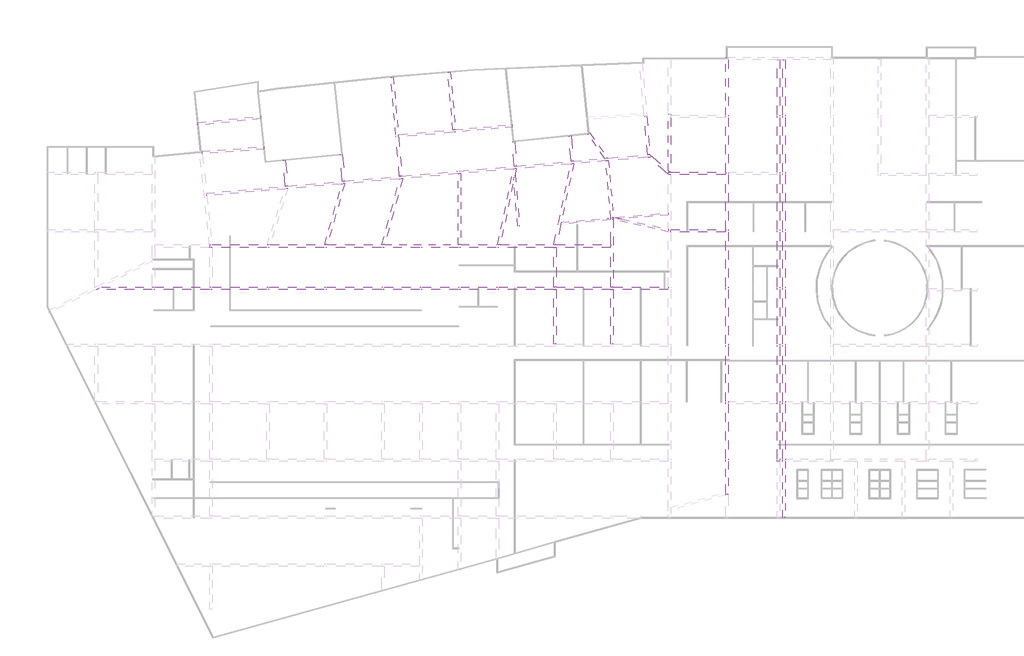
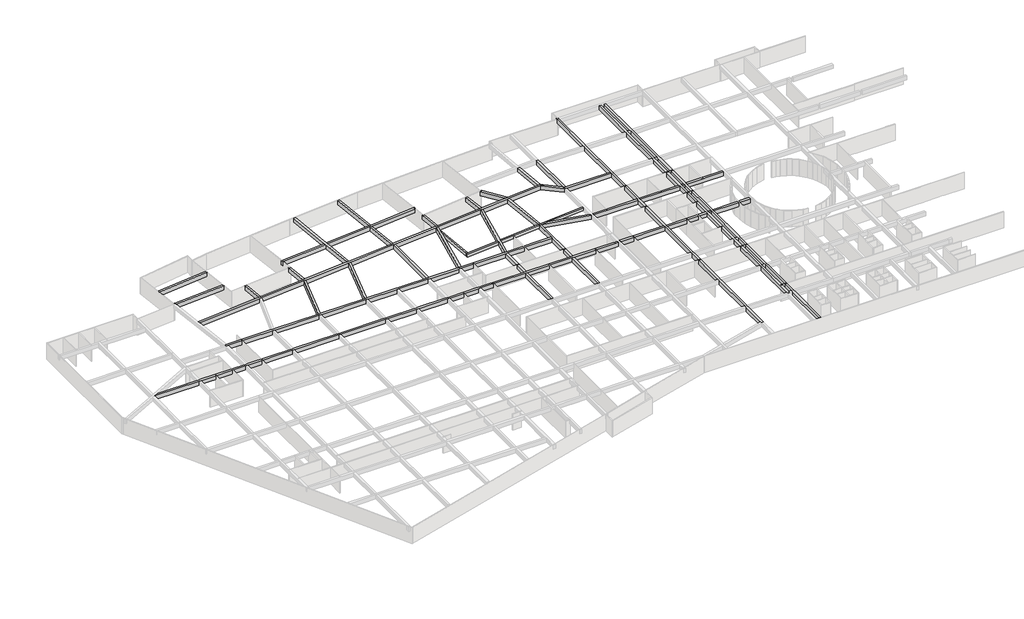
# One storey, part 7 of 8: 34 beams.
"""IFC4 building model written with IfcOpenShell, lengths in millimetres."""

import ifcopenshell
import ifcopenshell.guid

model = None  # the IFC model being written
_history = None  # IfcOwnerHistory: only IFC2X3 demands one
_inside = {}  # id of a spatial element -> (the spatial element, [elements in it])
_under = {}  # id of a project, library or spatial element -> (it, [spatial elements below it])
_declared = {}  # id of a project -> (the project, [libraries it declares])
_typed = {}  # id of a type object -> (the type object, [elements of that type])
_made_of = {}  # id of a material, layer set ... -> (it, [elements and type objects made of it])


def new_model(schema):
    """Start an empty IFC model of exactly this schema.

    Asked for "IFC4X3", IfcOpenShell would pick the latest addendum, in which some entities
    have other attributes; the version numbers below select the first issue.
    IFC2X3 requires an IfcOwnerHistory on every rooted entity: one is made here for all.
    """
    global model, _history
    if schema == "IFC4X3":
        model = ifcopenshell.file(schema_version=(4, 3, 0, 0))
    else:
        model = ifcopenshell.file(schema=schema)
    _inside.clear()
    _under.clear()
    _declared.clear()
    _typed.clear()
    _made_of.clear()
    _history = None
    if model.schema == "IFC2X3":
        org = make("IfcOrganization", Name="unknown")
        user = make(
            "IfcPersonAndOrganization",
            ThePerson=make("IfcPerson", FamilyName="unknown"),
            TheOrganization=org,
        )
        app = make(
            "IfcApplication",
            ApplicationDeveloper=org,
            Version="unknown",
            ApplicationFullName="unknown",
            ApplicationIdentifier="unknown",
        )
        _history = make(
            "IfcOwnerHistory",
            OwningUser=user,
            OwningApplication=app,
            ChangeAction="ADDED",
            CreationDate=0,
        )
    return model


def make(cls, **values):
    """One entity of the class cls with the attributes given. An attribute that is None is left unset."""
    return model.create_entity(
        cls, **{name: value for name, value in values.items() if value is not None}
    )


def rooted(cls, **values):
    """An entity with a GlobalId (a new one), such as an element, a storey or a relation."""
    return make(cls, GlobalId=ifcopenshell.guid.new(), OwnerHistory=_history, **values)


def si_unit(unit_type, name, prefix=None):
    """IfcSIUnit, for example si_unit("LENGTHUNIT", "METRE", prefix="MILLI")."""
    return make("IfcSIUnit", UnitType=unit_type, Prefix=prefix, Name=name)


def assignment(units):
    """IfcUnitAssignment: the units of a project."""
    return None if units is None else make("IfcUnitAssignment", Units=units)


def point(xyz):
    """IfcCartesianPoint."""
    return None if xyz is None else make("IfcCartesianPoint", Coordinates=xyz)


def direction(xyz):
    """IfcDirection."""
    return None if xyz is None else make("IfcDirection", DirectionRatios=xyz)


def frame(location, z_axis=None, x_axis=None):
    """IfcAxis2Placement3D, a coordinate frame: its origin and axes. An axis left out is left unset."""
    return make(
        "IfcAxis2Placement3D",
        Location=point(location),
        Axis=direction(z_axis),
        RefDirection=direction(x_axis),
    )


def origin():
    """The frame at (0, 0, 0) with its axes left unset."""
    return frame((0.0, 0.0, 0.0))


def place(relative_to, where):
    """IfcLocalPlacement: puts the frame where relative to a parent placement (None: the world)."""
    return make(
        "IfcLocalPlacement", PlacementRelTo=relative_to, RelativePlacement=where
    )


def context(
    kind, dimensions, precision=None, world=None, true_north=None, identifier=None
):
    """IfcGeometricRepresentationContext, for example the 3D "Model" context."""
    return make(
        "IfcGeometricRepresentationContext",
        ContextIdentifier=identifier,
        ContextType=kind,
        CoordinateSpaceDimension=dimensions,
        Precision=precision,
        WorldCoordinateSystem=world,
        TrueNorth=true_north,
    )


def project(units=None, contexts=None):
    """IfcProject with its units and contexts."""
    return rooted(
        "IfcProject",
        Name="project",
        RepresentationContexts=contexts,
        UnitsInContext=assignment(units),
    )


def spatial(cls, under=None, at=None, **own):
    """A site, building, storey or space (cls), placed at a placement, below another one or the project."""
    s = rooted(cls, ObjectPlacement=at, **own)
    if under is not None:
        _under.setdefault(under.id(), (under, []))[1].append(s)
    return s


def polyline(points):
    """IfcPolyline through the points."""
    return make("IfcPolyline", Points=[point(p) for p in points])


def outline(outer, holes=None, kind="AREA"):
    """IfcArbitraryClosedProfileDef: a profile drawn as a closed curve; with holes, ...WithVoids."""
    if holes is None:
        return make("IfcArbitraryClosedProfileDef", ProfileType=kind, OuterCurve=outer)
    return make(
        "IfcArbitraryProfileDefWithVoids",
        ProfileType=kind,
        OuterCurve=outer,
        InnerCurves=holes,
    )


def extrude(swept, where, along, depth):
    """IfcExtrudedAreaSolid: the profile swept, set in the frame where, extruded along a direction by depth."""
    return make(
        "IfcExtrudedAreaSolid",
        SweptArea=swept,
        Position=where,
        ExtrudedDirection=direction(along),
        Depth=depth,
    )


def faces_of(points, faces, orient=None, outer=None):
    """IfcFace entities. A face is a list of loops; a loop is a list of indices into points, from 0.

    orient and outer hold one flag for each loop. By default every Orientation is true, the
    first loop of a face is its IfcFaceOuterBound and the others are IfcFaceBound.
    """
    made = []
    for i, loops in enumerate(faces):
        bounds = []
        for j, loop in enumerate(loops):
            is_outer = j == 0 if outer is None else outer[i][j]
            bounds.append(
                make(
                    "IfcFaceOuterBound" if is_outer else "IfcFaceBound",
                    Bound=make("IfcPolyLoop", Polygon=[points[k] for k in loop]),
                    Orientation=True if orient is None else orient[i][j],
                )
            )
        made.append(make("IfcFace", Bounds=bounds))
    return made


def faceted_brep(points, faces, orient=None, outer=None, voids=None):
    """IfcFacetedBrep: a solid bounded by flat faces; with voids (closed shells), ...WithVoids."""
    shared = [point(p) for p in points]
    hull = make("IfcClosedShell", CfsFaces=faces_of(shared, faces, orient, outer))
    if voids is None:
        return make("IfcFacetedBrep", Outer=hull)
    return make(
        "IfcFacetedBrepWithVoids",
        Outer=hull,
        Voids=[
            make(cls, CfsFaces=faces_of(shared, fs, o, b)) for cls, fs, o, b in voids
        ],
    )


def shape(context_of_items, identifier, shape_type, items):
    """IfcShapeRepresentation: the items that make up one representation, for example the "Body"."""
    return make(
        "IfcShapeRepresentation",
        ContextOfItems=context_of_items,
        RepresentationIdentifier=identifier,
        RepresentationType=shape_type,
        Items=items,
    )


def source(mapping_origin, context_of_items, identifier, shape_type, items):
    """IfcRepresentationMap: a shape defined once, which mapped items show again and again."""
    return make(
        "IfcRepresentationMap",
        MappingOrigin=mapping_origin,
        MappedRepresentation=shape(context_of_items, identifier, shape_type, items),
    )


def transform(
    local_origin,
    x_axis=None,
    y_axis=None,
    z_axis=None,
    scale=None,
    scale2=None,
    scale3=None,
    uniform=True,
):
    """IfcCartesianTransformationOperator3D, or its non-uniform kind. x_axis, y_axis, z_axis: its Axis1, 2, 3."""
    if uniform:
        return make(
            "IfcCartesianTransformationOperator3D",
            Axis1=direction(x_axis),
            Axis2=direction(y_axis),
            LocalOrigin=point(local_origin),
            Scale=scale,
            Axis3=direction(z_axis),
        )
    return make(
        "IfcCartesianTransformationOperator3DnonUniform",
        Axis1=direction(x_axis),
        Axis2=direction(y_axis),
        LocalOrigin=point(local_origin),
        Scale=scale,
        Axis3=direction(z_axis),
        Scale2=scale2,
        Scale3=scale3,
    )


def mapped(mapping_source, mapping_target):
    """IfcMappedItem: shows the shape of a source again, moved by a transform."""
    return make(
        "IfcMappedItem", MappingSource=mapping_source, MappingTarget=mapping_target
    )


def made_of(thing, what):
    """Note that an element or type object is made of a material, layer set ...; save() writes the relation."""
    if what is not None:
        _made_of.setdefault(what.id(), (what, []))[1].append(thing)
    return thing


def element(
    cls,
    number,
    at=None,
    inside=None,
    cuts=None,
    type_object=None,
    material=None,
    context=None,
    identifier="Body",
    shape_type=None,
    held_by="IfcProductDefinitionShape",
    body=None,
    shapes=None,
    **own,
):
    """One element of the class cls, such as IfcWall. Its Tag is "e" and its number.

    at: its placement. inside: the storey or other place that contains it. cuts: it is an
    opening in that element (IfcRelVoidsElement). A single representation is given by context,
    identifier, shape_type and body (its items); several are given by shapes. held_by: the class
    of the entity that holds the representations. save() writes the other relations.
    """
    e = rooted(cls, Tag="e%d" % number, ObjectPlacement=at, **own)
    if body is not None:
        shapes = [shape(context, identifier, shape_type, body)]
    if shapes is not None:
        e.Representation = make(held_by, Representations=shapes)
    if inside is not None:
        _inside.setdefault(inside.id(), (inside, []))[1].append(e)
    if cuts is not None:
        rooted(
            "IfcRelVoidsElement", RelatingBuildingElement=cuts, RelatedOpeningElement=e
        )
    if type_object is not None:
        _typed.setdefault(type_object.id(), (type_object, []))[1].append(e)
    return made_of(e, material)


def aggregate(whole, parts):
    """IfcRelAggregates: a whole, such as a stair, and the parts it consists of."""
    return rooted("IfcRelAggregates", RelatingObject=whole, RelatedObjects=parts)


def save(model, path):
    """Write the relations noted so far, then the file.

    IfcRelAggregates (storeys below a building ...), IfcRelContainedInSpatialStructure (elements
    in a storey), IfcRelDefinesByType, IfcRelAssociatesMaterial and IfcRelDeclares: one each for
    every whole, place, type object, material and project.
    """
    for whole, parts in _under.values():
        aggregate(whole, parts)
    for where, things in _inside.values():
        rooted(
            "IfcRelContainedInSpatialStructure",
            RelatedElements=things,
            RelatingStructure=where,
        )
    for kind, things in _typed.values():
        rooted("IfcRelDefinesByType", RelatedObjects=things, RelatingType=kind)
    for what, things in _made_of.values():
        rooted("IfcRelAssociatesMaterial", RelatedObjects=things, RelatingMaterial=what)
    for by, libraries in _declared.values():
        rooted("IfcRelDeclares", RelatingContext=by, RelatedDefinitions=libraries)
    model.write(path)


def kl_beam_4b589649(model_context):
    return source(origin(), model_context, "Body", "SweptSolid", [
        extrude(outline(polyline([(4962.0, 200.0), (4962.0, -200.0), (-4962.0, -200.0), (-4962.0, 200.0), (4962.0, 200.0)])), frame((0.0, 0.0, -400.0), z_axis=(0.0, 0.0, 1.0), x_axis=(1.0, 0.0, 0.0)), (0.0, 0.0, 1.0), 800.0),
    ])


model = new_model("IFC4")

# Units and contexts
model_context = context("Model", 3, world=origin())
ifc_project = project(units=[si_unit("LENGTHUNIT", "METRE", prefix="MILLI")], contexts=[model_context])

# Site, building, storey
site = spatial("IfcSite", under=ifc_project)
building = spatial("IfcBuilding", under=site)
storey = spatial("IfcBuildingStorey", under=building, Name="户型图", Elevation=0.0)

# Beams
placement = place(None, origin())
element("IfcBeam", 1, ObjectType="混凝土 - 矩形梁 : KL_beam", at=placement, inside=storey, context=model_context, shape_type="Brep", body=[
    faceted_brep([(415153.8653576, -29460.9013816, 3300.0), (415153.8653576, -29460.9013816, 2500.0), (415553.8653576, -29460.9013816, 2500.0), (415553.8653576, -29460.9013816, 3300.0), (415553.8653576, -20661.3735096, 3300.0), (415553.8653576, -20261.3735096, 3300.0), (415553.8653576, -11661.3735096, 3300.0), (415553.8653576, -11261.3735096, 3300.0), (415553.8653576, -2661.3735096, 3300.0), (415553.8653576, -2261.3735096, 3300.0), (415553.8653576, 6338.6264904, 3300.0), (415553.8653576, 6738.6264904, 3300.0), (415553.8653576, 15338.6264904, 3300.0), (415553.8653576, 15738.6264904, 3300.0), (415553.8653576, 24338.6264659, 3300.0), (415553.8653576, 24738.6264659, 3300.0), (415553.8653576, 33338.6264904, 3300.0), (415553.8653576, 33738.6264904, 3300.0), (415553.8653576, 42435.5707464, 3300.0), (415153.8653576, 42435.5707464, 3300.0), (415153.8653576, 33738.6264904, 3300.0), (415153.8653576, 33338.6264904, 3300.0), (415153.8653576, 24738.6264659, 3300.0), (415153.8653576, 24338.6264659, 3300.0), (415153.8653576, 15738.6264904, 3300.0), (415153.8653576, 15338.6264904, 3300.0), (415153.8653576, 6738.6264904, 3300.0), (415153.8653576, 6338.6264904, 3300.0), (415153.8653576, -2261.3735096, 3300.0), (415153.8653576, -2661.3735096, 3300.0), (415153.8653576, -11261.3735096, 3300.0), (415153.8653576, -11661.3735096, 3300.0), (415153.8653576, -20261.3735096, 3300.0), (415153.8653576, -20661.3735096, 3300.0), (415553.8653576, -20661.3735096, 2500.0), (415553.8653576, -20261.3735096, 2500.0), (415553.8653576, -11661.3735096, 2500.0), (415553.8653576, -11261.3735096, 2500.0), (415553.8653576, -2661.3735096, 2500.0), (415553.8653576, -2261.3735096, 2500.0), (415553.8653576, 6338.6264904, 2500.0), (415553.8653576, 6738.6264904, 2500.0), (415553.8653576, 15338.6264904, 2500.0), (415553.8653576, 15738.6264904, 2500.0), (415553.8653576, 24338.6264659, 2500.0), (415553.8653576, 24738.6264659, 2500.0), (415553.8653576, 33338.6264904, 2500.0), (415553.8653576, 33738.6264904, 2500.0), (415553.8653576, 42435.5707464, 2500.0), (415153.8653576, -20661.3735096, 2500.0), (415153.8653576, -20261.3735096, 2500.0), (415153.8653576, -11661.3735096, 2500.0), (415153.8653576, -11261.3735096, 2500.0), (415153.8653576, -2661.3735096, 2500.0), (415153.8653576, -2261.3735096, 2500.0), (415153.8653576, 6338.6264904, 2500.0), (415153.8653576, 6738.6264904, 2500.0), (415153.8653576, 15338.6264904, 2500.0), (415153.8653576, 15738.6264904, 2500.0), (415153.8653576, 24338.6264659, 2500.0), (415153.8653576, 24738.6264659, 2500.0), (415153.8653576, 33338.6264904, 2500.0), (415153.8653576, 33738.6264904, 2500.0), (415153.8653576, 42435.5707464, 2500.0)], [[[0, 1, 2, 3]], [[0, 3, 4, 5, 6, 7, 8, 9, 10, 11, 12, 13, 14, 15, 16, 17, 18, 19, 20, 21, 22, 23, 24, 25, 26, 27, 28, 29, 30, 31, 32, 33]], [[3, 2, 34, 35, 36, 37, 38, 39, 40, 41, 42, 43, 44, 45, 46, 47, 48, 18, 17, 16, 15, 14, 13, 12, 11, 10, 9, 8, 7, 6, 5, 4]], [[2, 1, 49, 50, 51, 52, 53, 54, 55, 56, 57, 58, 59, 60, 61, 62, 63, 48, 47, 46, 45, 44, 43, 42, 41, 40, 39, 38, 37, 36, 35, 34]], [[1, 0, 33, 32, 31, 30, 29, 28, 27, 26, 25, 24, 23, 22, 21, 20, 19, 63, 62, 61, 60, 59, 58, 57, 56, 55, 54, 53, 52, 51, 50, 49]], [[19, 18, 48, 63]]]),
])
element("IfcBeam", 2, ObjectType="混凝土 - 矩形梁 : KL_beam", at=placement, inside=storey, context=model_context, shape_type="Brep", body=[
    faceted_brep([(414253.8653576, -20661.3735124, 3300.0), (414653.8653576, -20661.3735124, 3300.0), (414653.8653576, -20261.3735096, 3300.0), (414653.8653576, -11661.3735096, 3300.0), (414653.8653576, -11261.3735096, 3300.0), (414653.8653576, -2661.3735096, 3300.0), (414653.8653576, -2261.3735096, 3300.0), (414653.8653576, 6338.6264904, 3300.0), (414653.8653576, 6738.6264904, 3300.0), (414653.8653576, 15338.6264904, 3300.0), (414653.8653576, 15738.6264904, 3300.0), (414653.8653576, 24338.6264659, 3300.0), (414653.8653576, 24738.6264659, 3300.0), (414653.8653576, 33338.6264904, 3300.0), (414653.8653576, 33738.6264904, 3300.0), (414653.8653576, 42435.5707464, 3300.0), (414253.8653576, 42435.5707464, 3300.0), (414253.8653576, 33738.6264904, 3300.0), (414253.8653576, 33338.6264904, 3300.0), (414253.8653576, 24738.6264659, 3300.0), (414253.8653576, 24338.6264659, 3300.0), (414253.8653576, 15738.6264904, 3300.0), (414253.8653576, 15338.6264904, 3300.0), (414253.8653576, 6738.6264904, 3300.0), (414253.8653576, 6338.6264904, 3300.0), (414253.8653576, -2261.3735096, 3300.0), (414253.8653576, -2661.3735096, 3300.0), (414253.8653576, -11261.3735096, 3300.0), (414253.8653576, -11661.3735096, 3300.0), (414253.8653576, -20261.3735124, 3300.0), (414253.8653576, -20661.3735124, 2500.0), (414253.8653576, 42435.5707464, 2500.0), (414253.8653576, 33738.6264904, 2500.0), (414253.8653576, 33338.6264904, 2500.0), (414253.8653576, 24738.6264659, 2500.0), (414253.8653576, 24338.6264659, 2500.0), (414253.8653576, 15738.6264904, 2500.0), (414253.8653576, 15338.6264904, 2500.0), (414253.8653576, 6738.6264904, 2500.0), (414253.8653576, 6338.6264904, 2500.0), (414253.8653576, -2261.3735096, 2500.0), (414253.8653576, -2661.3735096, 2500.0), (414253.8653576, -11261.3735096, 2500.0), (414253.8653576, -11661.3735096, 2500.0), (414253.8653576, -20261.3735124, 2500.0), (414653.8653576, -20661.3735124, 2500.0), (414653.8653576, 42435.5707464, 2500.0), (414653.8653576, 33738.6264904, 2500.0), (414653.8653576, 33338.6264904, 2500.0), (414653.8653576, 24738.6264659, 2500.0), (414653.8653576, 24338.6264659, 2500.0), (414653.8653576, 15738.6264904, 2500.0), (414653.8653576, 15338.6264904, 2500.0), (414653.8653576, 6738.6264904, 2500.0), (414653.8653576, 6338.6264904, 2500.0), (414653.8653576, -2261.3735096, 2500.0), (414653.8653576, -2661.3735096, 2500.0), (414653.8653576, -11261.3735096, 2500.0), (414653.8653576, -11661.3735096, 2500.0), (414653.8653576, -20261.3735096, 2500.0)], [[[0, 1, 2, 3, 4, 5, 6, 7, 8, 9, 10, 11, 12, 13, 14, 15, 16, 17, 18, 19, 20, 21, 22, 23, 24, 25, 26, 27, 28, 29]], [[30, 0, 29, 28, 27, 26, 25, 24, 23, 22, 21, 20, 19, 18, 17, 16, 31, 32, 33, 34, 35, 36, 37, 38, 39, 40, 41, 42, 43, 44]], [[45, 30, 44, 43, 42, 41, 40, 39, 38, 37, 36, 35, 34, 33, 32, 31, 46, 47, 48, 49, 50, 51, 52, 53, 54, 55, 56, 57, 58, 59]], [[1, 45, 59, 58, 57, 56, 55, 54, 53, 52, 51, 50, 49, 48, 47, 46, 15, 14, 13, 12, 11, 10, 9, 8, 7, 6, 5, 4, 3, 2]], [[16, 15, 46, 31]], [[1, 0, 30, 45]]]),
])
element("IfcBeam", 3, ObjectType="混凝土 - 矩形梁 : KL_beam", at=placement, inside=storey, context=model_context, shape_type="Brep", body=[
    faceted_brep([(406553.8653576, 42835.5707464, 3300.0), (406153.8653576, 42835.5707464, 3300.0), (406153.8653576, 33738.6264904, 3300.0), (406153.8653576, 33338.6264904, 3300.0), (406153.8653576, 24738.6264659, 3300.0), (406153.8653576, 24338.6264659, 3300.0), (406153.8653576, 15738.6264904, 3300.0), (406153.8653576, 15338.6264904, 3300.0), (406153.8653576, 6738.6264904, 3300.0), (406153.8653576, 6338.6264904, 3300.0), (406153.8653576, -2261.3735096, 3300.0), (406153.8653576, -2661.3735096, 3300.0), (406153.8653576, -11261.3735096, 3300.0), (406153.8653576, -11661.3735096, 3300.0), (406153.8653576, -20261.3735124, 3300.0), (406153.8653576, -20661.3735124, 3300.0), (406153.8653576, -25536.5369512, 3300.0), (406153.8653576, -25951.6823221, 3300.0), (406553.8653576, -25840.571211, 3300.0), (406553.8653576, -20661.3735124, 3300.0), (406553.8653576, -20261.3735124, 3300.0), (406553.8653576, -11661.3735096, 3300.0), (406553.8653576, -11261.3735096, 3300.0), (406553.8653576, -2661.3735096, 3300.0), (406553.8653576, -2261.3735096, 3300.0), (406553.8653576, 6338.6264904, 3300.0), (406553.8653576, 6738.6264904, 3300.0), (406553.8653576, 15338.6264904, 3300.0), (406553.8653576, 15738.6264904, 3300.0), (406553.8653576, 24338.6264659, 3300.0), (406553.8653576, 24738.6264659, 3300.0), (406553.8653576, 33338.6264904, 3300.0), (406553.8653576, 33738.6264904, 3300.0), (406553.8653576, 42435.5707464, 3300.0), (406553.8653576, 42835.5707464, 2500.0), (406553.8653576, -25840.571211, 2500.0), (406553.8653576, -20661.3735124, 2500.0), (406553.8653576, -20261.3735124, 2500.0), (406553.8653576, -11661.3735096, 2500.0), (406553.8653576, -11261.3735096, 2500.0), (406553.8653576, -2661.3735096, 2500.0), (406553.8653576, -2261.3735096, 2500.0), (406553.8653576, 6338.6264904, 2500.0), (406553.8653576, 6738.6264904, 2500.0), (406553.8653576, 15338.6264904, 2500.0), (406553.8653576, 15738.6264904, 2500.0), (406553.8653576, 24338.6264659, 2500.0), (406553.8653576, 24738.6264659, 2500.0), (406553.8653576, 33338.6264904, 2500.0), (406553.8653576, 33738.6264904, 2500.0), (406553.8653576, 42435.5707464, 2500.0), (406153.8653576, 42835.5707464, 2500.0), (406153.8653576, -25951.6823221, 2500.0), (406153.8653576, -25536.5369512, 2500.0), (406153.8653576, -20661.3735124, 2500.0), (406153.8653576, -20261.3735124, 2500.0), (406153.8653576, -11661.3735096, 2500.0), (406153.8653576, -11261.3735096, 2500.0), (406153.8653576, -2661.3735096, 2500.0), (406153.8653576, -2261.3735096, 2500.0), (406153.8653576, 6338.6264904, 2500.0), (406153.8653576, 6738.6264904, 2500.0), (406153.8653576, 15338.6264904, 2500.0), (406153.8653576, 15738.6264904, 2500.0), (406153.8653576, 24338.6264659, 2500.0), (406153.8653576, 24738.6264659, 2500.0), (406153.8653576, 33338.6264904, 2500.0), (406153.8653576, 33738.6264904, 2500.0)], [[[0, 1, 2, 3, 4, 5, 6, 7, 8, 9, 10, 11, 12, 13, 14, 15, 16, 17, 18, 19, 20, 21, 22, 23, 24, 25, 26, 27, 28, 29, 30, 31, 32, 33]], [[34, 0, 33, 32, 31, 30, 29, 28, 27, 26, 25, 24, 23, 22, 21, 20, 19, 18, 35, 36, 37, 38, 39, 40, 41, 42, 43, 44, 45, 46, 47, 48, 49, 50]], [[51, 34, 50, 49, 48, 47, 46, 45, 44, 43, 42, 41, 40, 39, 38, 37, 36, 35, 52, 53, 54, 55, 56, 57, 58, 59, 60, 61, 62, 63, 64, 65, 66, 67]], [[1, 51, 67, 66, 65, 64, 63, 62, 61, 60, 59, 58, 57, 56, 55, 54, 53, 52, 17, 16, 15, 14, 13, 12, 11, 10, 9, 8, 7, 6, 5, 4, 3, 2]], [[1, 0, 34, 51]], [[18, 17, 52, 35]]]),
])
element("IfcBeam", 4, ObjectType="混凝土 - 矩形梁 : KL_beam", at=placement, inside=storey, context=model_context, shape_type="Brep", body=[
    faceted_brep([(397153.8653576, 24738.6264659, 3300.0), (397153.8653576, 24446.9357612, 3300.0), (397153.8653576, 24338.6264659, 3300.0), (397553.8653576, 24338.6264659, 3300.0), (406153.8653576, 24338.6264659, 3300.0), (406153.8653576, 24738.6264659, 3300.0), (397553.8653576, 24738.6264659, 3300.0), (397428.1284682, 24738.6264659, 3300.0), (397153.8653576, 24738.6264659, 2500.0), (406153.8653576, 24738.6264659, 2500.0), (397553.8653576, 24738.6264659, 2500.0), (397428.1284682, 24738.6264659, 2500.0), (397153.8653576, 24338.6264659, 2500.0), (397153.8653576, 24446.9357612, 2500.0), (406153.8653576, 24338.6264659, 2500.0), (397553.8653576, 24338.6264659, 2500.0)], [[[0, 1, 2, 3, 4, 5, 6, 7]], [[8, 0, 7, 6, 5, 9, 10, 11]], [[12, 13, 8, 11, 10, 9, 14, 15]], [[2, 12, 15, 14, 4, 3]], [[5, 4, 14, 9]], [[2, 1, 0, 8, 13, 12]]]),
])
element("IfcBeam", 5, ObjectType="混凝土 - 矩形梁 : KL_beam", at=placement, inside=storey, context=model_context, shape_type="Brep", body=[
    faceted_brep([(422653.8653576, 6338.6264904, 3300.0), (422653.8653576, 6738.6264904, 3300.0), (415553.8653576, 6738.6264904, 3300.0), (415553.8653576, 6338.6264904, 3300.0), (422653.8653576, 6338.6264904, 2500.0), (415553.8653576, 6338.6264904, 2500.0), (422653.8653576, 6738.6264904, 2500.0), (415553.8653576, 6738.6264904, 2500.0)], [[[0, 1, 2, 3]], [[4, 0, 3, 5]], [[6, 4, 5, 7]], [[1, 6, 7, 2]], [[1, 0, 4, 6]], [[3, 2, 7, 5]]]),
    faceted_brep([(415153.8653576, 6738.6264904, 3300.0), (415153.8653576, 6338.6264904, 3300.0), (415153.8653576, 6338.6264904, 2500.0), (415153.8653576, 6738.6264904, 2500.0), (414653.8653576, 6738.6264904, 3300.0), (414653.8653576, 6338.6264904, 3300.0), (414653.8653576, 6338.6264904, 2500.0), (414653.8653576, 6738.6264904, 2500.0)], [[[0, 1, 2, 3]], [[1, 0, 4, 5]], [[2, 1, 5, 6]], [[3, 2, 6, 7]], [[0, 3, 7, 4]], [[5, 4, 7, 6]]]),
    faceted_brep([(414253.8653576, 6738.6264904, 3300.0), (414253.8653576, 6338.6264904, 3300.0), (414253.8653576, 6338.6264904, 2500.0), (414253.8653576, 6738.6264904, 2500.0), (406553.8653576, 6738.6264904, 3300.0), (406553.8653576, 6338.6264904, 3300.0), (406553.8653576, 6338.6264904, 2500.0), (406553.8653576, 6738.6264904, 2500.0)], [[[0, 1, 2, 3]], [[1, 0, 4, 5]], [[2, 1, 5, 6]], [[3, 2, 6, 7]], [[0, 3, 7, 4]], [[5, 4, 7, 6]]]),
    faceted_brep([(406153.8653576, 6738.6264904, 3300.0), (406153.8653576, 6338.6264904, 3300.0), (406153.8653576, 6338.6264904, 2500.0), (406153.8653576, 6738.6264904, 2500.0), (397553.8653576, 6738.6264904, 3300.0), (397553.8653576, 6338.6264904, 3300.0), (397553.8653576, 6338.6264904, 2500.0), (397553.8653576, 6738.6264904, 2500.0)], [[[0, 1, 2, 3]], [[1, 0, 4, 5]], [[2, 1, 5, 6]], [[3, 2, 6, 7]], [[0, 3, 7, 4]], [[5, 4, 7, 6]]]),
    faceted_brep([(397153.8653576, 6738.6264904, 3300.0), (397153.8653576, 6338.6264904, 3300.0), (397153.8653576, 6338.6264904, 2500.0), (397153.8653576, 6738.6264904, 2500.0), (388553.8653576, 6738.6264904, 3300.0), (388153.8653576, 6738.6264904, 3300.0), (379553.8653576, 6738.6264904, 3300.0), (379153.8653576, 6738.6264904, 3300.0), (370553.8653576, 6738.6264904, 3300.0), (370153.8653576, 6738.6264904, 3300.0), (364553.8653576, 6738.6264904, 3300.0), (364153.8653576, 6738.6264904, 3300.0), (358553.8653576, 6738.6264904, 3300.0), (358153.8653576, 6738.6264904, 3300.0), (352553.8653576, 6738.6264904, 3300.0), (352153.8653576, 6738.6264904, 3300.0), (343553.8653576, 6738.6264904, 3300.0), (343153.8653576, 6738.6264904, 3300.0), (334553.8653576, 6738.6264904, 3300.0), (334153.8653576, 6738.6264904, 3300.0), (325553.8653576, 6738.6264904, 3300.0), (325153.8653576, 6738.6264904, 3300.0), (316553.8653576, 6738.6264904, 3300.0), (316153.8653576, 6738.6264904, 3300.0), (308201.0789512, 6738.6264904, 3300.0), (307401.078951, 6338.6264904, 3300.0), (307553.8653555, 6338.6264904, 3300.0), (316153.8653576, 6338.6264904, 3300.0), (316553.8653576, 6338.6264904, 3300.0), (325153.8653576, 6338.6264904, 3300.0), (325553.8653576, 6338.6264904, 3300.0), (334153.8653576, 6338.6264904, 3300.0), (334553.8653576, 6338.6264904, 3300.0), (343153.8653576, 6338.6264904, 3300.0), (343553.8653576, 6338.6264904, 3300.0), (352153.8653576, 6338.6264904, 3300.0), (352553.8653576, 6338.6264904, 3300.0), (358153.8653576, 6338.6264904, 3300.0), (358553.8653576, 6338.6264904, 3300.0), (364153.8653576, 6338.6264904, 3300.0), (364553.8653576, 6338.6264904, 3300.0), (370153.8653576, 6338.6264904, 3300.0), (370553.8653576, 6338.6264904, 3300.0), (379153.8653576, 6338.6264904, 3300.0), (379553.8653576, 6338.6264904, 3300.0), (388153.8653576, 6338.6264904, 3300.0), (388553.8653576, 6338.6264904, 3300.0), (307401.078951, 6338.6264904, 2500.0), (307553.8653555, 6338.6264904, 2500.0), (316153.8653576, 6338.6264904, 2500.0), (316553.8653576, 6338.6264904, 2500.0), (325153.8653576, 6338.6264904, 2500.0), (325553.8653576, 6338.6264904, 2500.0), (334153.8653576, 6338.6264904, 2500.0), (334553.8653576, 6338.6264904, 2500.0), (343153.8653576, 6338.6264904, 2500.0), (343553.8653576, 6338.6264904, 2500.0), (352153.8653576, 6338.6264904, 2500.0), (352553.8653576, 6338.6264904, 2500.0), (358153.8653576, 6338.6264904, 2500.0), (358553.8653576, 6338.6264904, 2500.0), (364153.8653576, 6338.6264904, 2500.0), (364553.8653576, 6338.6264904, 2500.0), (370153.8653576, 6338.6264904, 2500.0), (370553.8653576, 6338.6264904, 2500.0), (379153.8653576, 6338.6264904, 2500.0), (379553.8653576, 6338.6264904, 2500.0), (388153.8653576, 6338.6264904, 2500.0), (388553.8653576, 6338.6264904, 2500.0), (308201.0789512, 6738.6264904, 2500.0), (316153.8653576, 6738.6264904, 2500.0), (316553.8653576, 6738.6264904, 2500.0), (325153.8653576, 6738.6264904, 2500.0), (325553.8653576, 6738.6264904, 2500.0), (334153.8653576, 6738.6264904, 2500.0), (334553.8653576, 6738.6264904, 2500.0), (343153.8653576, 6738.6264904, 2500.0), (343553.8653576, 6738.6264904, 2500.0), (352153.8653576, 6738.6264904, 2500.0), (352553.8653576, 6738.6264904, 2500.0), (358153.8653576, 6738.6264904, 2500.0), (358553.8653576, 6738.6264904, 2500.0), (364153.8653576, 6738.6264904, 2500.0), (364553.8653576, 6738.6264904, 2500.0), (370153.8653576, 6738.6264904, 2500.0), (370553.8653576, 6738.6264904, 2500.0), (379153.8653576, 6738.6264904, 2500.0), (379553.8653576, 6738.6264904, 2500.0), (388153.8653576, 6738.6264904, 2500.0), (388553.8653576, 6738.6264904, 2500.0)], [[[0, 1, 2, 3]], [[1, 0, 4, 5, 6, 7, 8, 9, 10, 11, 12, 13, 14, 15, 16, 17, 18, 19, 20, 21, 22, 23, 24, 25, 26, 27, 28, 29, 30, 31, 32, 33, 34, 35, 36, 37, 38, 39, 40, 41, 42, 43, 44, 45, 46]], [[2, 1, 46, 45, 44, 43, 42, 41, 40, 39, 38, 37, 36, 35, 34, 33, 32, 31, 30, 29, 28, 27, 26, 25, 47, 48, 49, 50, 51, 52, 53, 54, 55, 56, 57, 58, 59, 60, 61, 62, 63, 64, 65, 66, 67, 68]], [[3, 2, 68, 67, 66, 65, 64, 63, 62, 61, 60, 59, 58, 57, 56, 55, 54, 53, 52, 51, 50, 49, 48, 47, 69, 70, 71, 72, 73, 74, 75, 76, 77, 78, 79, 80, 81, 82, 83, 84, 85, 86, 87, 88, 89]], [[0, 3, 89, 88, 87, 86, 85, 84, 83, 82, 81, 80, 79, 78, 77, 76, 75, 74, 73, 72, 71, 70, 69, 24, 23, 22, 21, 20, 19, 18, 17, 16, 15, 14, 13, 12, 11, 10, 9, 8, 7, 6, 5, 4]], [[25, 24, 69, 47]]]),
])
element("IfcBeam", 6, ObjectType="混凝土 - 矩形梁 : KL_beam", at=placement, inside=storey, context=model_context, shape_type="SweptSolid", body=[
    extrude(outline(polyline([(422653.8653576, 15738.6264904), (422653.8653576, 15338.6264904), (415553.8653576, 15338.6264904), (415553.8653576, 15738.6264904), (422653.8653576, 15738.6264904)])), frame((0.0, 0.0, 2500.0), z_axis=(0.0, 0.0, 1.0), x_axis=(1.0, 0.0, 0.0)), (0.0, 0.0, 1.0), 800.0),
    extrude(outline(polyline([(397553.8653576, 15338.6264904), (397553.8653576, 15738.6264904), (406153.8653576, 15738.6264904), (406153.8653576, 15338.6264904), (397553.8653576, 15338.6264904)])), frame((0.0, 0.0, 2500.0), z_axis=(0.0, 0.0, 1.0), x_axis=(1.0, 0.0, 0.0)), (0.0, 0.0, 1.0), 800.0),
    extrude(outline(polyline([(415153.8653576, 15738.6264904), (415153.8653576, 15338.6264904), (414653.8653576, 15338.6264904), (414653.8653576, 15738.6264904), (415153.8653576, 15738.6264904)])), frame((0.0, 0.0, 2500.0), z_axis=(0.0, 0.0, 1.0), x_axis=(1.0, 0.0, 0.0)), (0.0, 0.0, 1.0), 800.0),
    extrude(outline(polyline([(414253.8653576, 15738.6264904), (414253.8653576, 15338.6264904), (406553.8653576, 15338.6264904), (406553.8653576, 15738.6264904), (414253.8653576, 15738.6264904)])), frame((0.0, 0.0, 2500.0), z_axis=(0.0, 0.0, 1.0), x_axis=(1.0, 0.0, 0.0)), (0.0, 0.0, 1.0), 800.0),
])
element("IfcBeam", 7, ObjectType="混凝土 - 矩形梁 : KL_beam", at=placement, inside=storey, context=model_context, shape_type="Brep", body=[
    faceted_brep([(388153.8653576, 6738.6264904, 3300.0), (388553.8653576, 6738.6264904, 3300.0), (388553.8653576, 17289.3032923, 3300.0), (388553.8653576, 17298.9593378, 3300.0), (388153.8653576, 17264.1311188, 3300.0), (388153.8653576, 13338.6264904, 3300.0), (388153.8653576, 12938.6264904, 3300.0), (388553.8653576, 6738.6264904, 2500.0), (388553.8653576, 17289.3032923, 2500.0), (388553.8653576, 17600.0943826, 2500.0), (388553.8653576, 17600.0943826, 2700.0), (388553.8653576, 17298.9593378, 2700.0), (388153.8653576, 6738.6264904, 2500.0), (388153.8653576, 12938.6264904, 2500.0), (388153.8653576, 13338.6264904, 2500.0), (388153.8653576, 17378.1921818, 2500.0), (388153.8653576, 17565.2661636, 2500.0), (388549.2864631, 17599.6956957, 2500.0), (388153.8653576, 17264.1311188, 2700.0), (388153.8653576, 17378.1921818, 2700.0), (388153.8653576, 17565.2661636, 2700.0)], [[[0, 1, 2, 3, 4, 5, 6]], [[1, 7, 8, 9, 10, 11, 3, 2]], [[7, 12, 13, 14, 15, 16, 17, 9, 8]], [[12, 0, 6, 5, 4, 18, 19, 20, 16, 15, 14, 13]], [[1, 0, 12, 7]], [[9, 17, 16, 20, 10]], [[11, 18, 4, 3]], [[18, 11, 10, 20, 19]]]),
])
element("IfcBeam", 8, ObjectType="混凝土 - 矩形梁 : KL_beam", at=placement, inside=storey, context=model_context, shape_type="SweptSolid", body=[
    extrude(outline(polyline([(379553.8653576, 6738.6264904), (379153.8653576, 6738.6264904), (379153.8653576, 12938.6264904), (379553.8653576, 12938.6264904), (379553.8653576, 6738.6264904)])), frame((0.0, 0.0, 2500.0), z_axis=(0.0, 0.0, 1.0), x_axis=(1.0, 0.0, 0.0)), (0.0, 0.0, 1.0), 800.0),
])
element("IfcBeam", 9, ObjectType="混凝土 - 矩形梁 : KL_beam", at=placement, inside=storey, context=model_context, shape_type="Brep", body=[
    faceted_brep([(325153.8653576, 13338.6264904, 3300.0), (325153.8653576, 12938.6264904, 3300.0), (325553.8653576, 12938.6264904, 3300.0), (334153.8653576, 12938.6264904, 3300.0), (334553.8653576, 12938.6264904, 3300.0), (343153.8653576, 12938.6264904, 3300.0), (343553.8653576, 12938.6264904, 3300.0), (352153.8653576, 12938.6264904, 3300.0), (352553.8653576, 12938.6264904, 3300.0), (358153.8653576, 12938.6264904, 3300.0), (358553.8653576, 12938.6264904, 3300.0), (364153.8653576, 12938.6264904, 3300.0), (364553.8653576, 12938.6264904, 3300.0), (370153.8653576, 12938.6264904, 3300.0), (370553.8653576, 12938.6264904, 3300.0), (379153.8653576, 12938.6264904, 3300.0), (379553.8653576, 12938.6264904, 3300.0), (388153.8653576, 12938.6264904, 3300.0), (388153.8653576, 13338.6264904, 3300.0), (379600.8447889, 13338.6264904, 3300.0), (379191.908551, 13338.6264904, 3300.0), (370799.39661, 13338.6264904, 3300.0), (370390.9533063, 13338.6264904, 3300.0), (370153.8653576, 13338.6264904, 3300.0), (364553.8653576, 13338.6264904, 3300.0), (364153.8653576, 13338.6264904, 3300.0), (352615.456713, 13338.6264904, 3300.0), (352200.9551059, 13338.6264904, 3300.0), (343618.9569006, 13338.6264904, 3300.0), (343202.974086, 13338.6264904, 3300.0), (334626.1752673, 13338.6264904, 3300.0), (334206.9738984, 13338.6264904, 3300.0), (325533.9679202, 13338.6264904, 3300.0), (325153.8653576, 13338.6264904, 2500.0), (388153.8653576, 13338.6264904, 2500.0), (379600.8447889, 13338.6264904, 2500.0), (379191.908551, 13338.6264904, 2500.0), (370799.39661, 13338.6264904, 2500.0), (370390.9533063, 13338.6264904, 2500.0), (370153.8653576, 13338.6264904, 2500.0), (364553.8653576, 13338.6264904, 2500.0), (364153.8653576, 13338.6264904, 2500.0), (352615.456713, 13338.6264904, 2500.0), (352200.9551059, 13338.6264904, 2500.0), (343618.9569006, 13338.6264904, 2500.0), (343202.974086, 13338.6264904, 2500.0), (334626.1752673, 13338.6264904, 2500.0), (334206.9738984, 13338.6264904, 2500.0), (325533.9679202, 13338.6264904, 2500.0), (325153.8653576, 12938.6264904, 2500.0), (388153.8653576, 12938.6264904, 2500.0), (379553.8653576, 12938.6264904, 2500.0), (379153.8653576, 12938.6264904, 2500.0), (370553.8653576, 12938.6264904, 2500.0), (370153.8653576, 12938.6264904, 2500.0), (364553.8653576, 12938.6264904, 2500.0), (364153.8653576, 12938.6264904, 2500.0), (358553.8653576, 12938.6264904, 2500.0), (358153.8653576, 12938.6264904, 2500.0), (352553.8653576, 12938.6264904, 2500.0), (352153.8653576, 12938.6264904, 2500.0), (343553.8653576, 12938.6264904, 2500.0), (343153.8653576, 12938.6264904, 2500.0), (334553.8653576, 12938.6264904, 2500.0), (334153.8653576, 12938.6264904, 2500.0), (325553.8653576, 12938.6264904, 2500.0)], [[[0, 1, 2, 3, 4, 5, 6, 7, 8, 9, 10, 11, 12, 13, 14, 15, 16, 17, 18, 19, 20, 21, 22, 23, 24, 25, 26, 27, 28, 29, 30, 31, 32]], [[33, 0, 32, 31, 30, 29, 28, 27, 26, 25, 24, 23, 22, 21, 20, 19, 18, 34, 35, 36, 37, 38, 39, 40, 41, 42, 43, 44, 45, 46, 47, 48]], [[49, 33, 48, 47, 46, 45, 44, 43, 42, 41, 40, 39, 38, 37, 36, 35, 34, 50, 51, 52, 53, 54, 55, 56, 57, 58, 59, 60, 61, 62, 63, 64, 65]], [[1, 49, 65, 64, 63, 62, 61, 60, 59, 58, 57, 56, 55, 54, 53, 52, 51, 50, 17, 16, 15, 14, 13, 12, 11, 10, 9, 8, 7, 6, 5, 4, 3, 2]], [[18, 17, 50, 34]], [[1, 0, 33, 49]]]),
])
element("IfcBeam", 10, ObjectType="混凝土 - 矩形梁 : KL_beam", at=placement, inside=storey, context=model_context, shape_type="Brep", body=[
    faceted_brep([(394612.9521543, 27163.6090151, 3300.0), (394315.3342126, 27419.9760183, 3300.0), (394189.7945144, 27528.1154538, 3300.0), (393906.5136104, 27503.3315861, 3300.0), (387645.6838003, 26955.5799534, 3300.0), (387185.131228, 26915.2868244, 3300.0), (382324.182255, 26490.0088953, 3300.0), (381925.6445092, 26455.1413605, 3300.0), (373384.9028298, 25707.9232855, 3300.0), (372986.4249505, 25673.0609884, 3300.0), (364319.6200132, 24914.8138074, 3300.0), (363921.142134, 24879.9515103, 3300.0), (355353.8677558, 24130.4121249, 3300.0), (354955.3898765, 24095.5498278, 3300.0), (346386.1102387, 23345.8350049, 3300.0), (345987.6137498, 23310.9710796, 3300.0), (337422.2742287, 22561.6009723, 3300.0), (337023.7963495, 22526.7386752, 3300.0), (324682.7246887, 21447.0348091, 3300.0), (324724.4945588, 21049.1612642, 3300.0), (336960.2296074, 22119.6493709, 3300.0), (337391.2547421, 22157.3591839, 3300.0), (345934.1123721, 22904.7623806, 3300.0), (346360.7518178, 22942.0884955, 3300.0), (354990.254449, 23697.0721476, 3300.0), (355015.985011, 23699.3232801, 3300.0), (355440.5796188, 23736.4704949, 3300.0), (364153.8653576, 24498.7842191, 3300.0), (364553.8653576, 24533.7796845, 3300.0), (372853.2650418, 25259.8830709, 3300.0), (373269.2249952, 25296.2748513, 3300.0), (381893.9734922, 26050.8425706, 3300.0), (382310.6585256, 26087.2977873, 3300.0), (387366.4908773, 26529.6258027, 3300.0), (387764.9687566, 26564.4880998, 3300.0), (394056.572883, 27114.9321363, 3300.0), (394612.9521543, 27163.6090151, 2500.0), (324724.4945588, 21049.1612642, 2500.0), (336960.2296074, 22119.6493709, 2500.0), (337391.2547421, 22157.3591839, 2500.0), (345934.1123721, 22904.7623806, 2500.0), (346360.7518178, 22942.0884955, 2500.0), (354990.254449, 23697.0721476, 2500.0), (355015.985011, 23699.3232801, 2500.0), (355440.5796188, 23736.4704949, 2500.0), (364153.8653576, 24498.7842191, 2500.0), (364553.8653576, 24533.7796845, 2500.0), (372853.2650418, 25259.8830709, 2500.0), (373269.2249952, 25296.2748513, 2500.0), (381893.9734922, 26050.8425706, 2500.0), (382310.6585256, 26087.2977873, 2500.0), (387366.4908773, 26529.6258027, 2500.0), (387764.9687566, 26564.4880998, 2500.0), (394056.572883, 27114.9321363, 2500.0), (394189.7945144, 27528.1154538, 2500.0), (394315.3342126, 27419.9760183, 2500.0), (324682.7246887, 21447.0348091, 2500.0), (337023.7963495, 22526.7386752, 2500.0), (337422.2742287, 22561.6009723, 2500.0), (345987.6137498, 23310.9710796, 2500.0), (346386.1102387, 23345.8350049, 2500.0), (354955.3898765, 24095.5498278, 2500.0), (355353.8677558, 24130.4121249, 2500.0), (363921.142134, 24879.9515103, 2500.0), (364319.6200132, 24914.8138074, 2500.0), (372986.4249505, 25673.0609884, 2500.0), (373384.9028298, 25707.9232855, 2500.0), (381925.6445092, 26455.1413605, 2500.0), (382324.182255, 26490.0088953, 2500.0), (387185.131228, 26915.2868244, 2500.0), (387645.6838003, 26955.5799534, 2500.0), (393906.5136104, 27503.3315861, 2500.0)], [[[0, 1, 2, 3, 4, 5, 6, 7, 8, 9, 10, 11, 12, 13, 14, 15, 16, 17, 18, 19, 20, 21, 22, 23, 24, 25, 26, 27, 28, 29, 30, 31, 32, 33, 34, 35]], [[36, 0, 35, 34, 33, 32, 31, 30, 29, 28, 27, 26, 25, 24, 23, 22, 21, 20, 19, 37, 38, 39, 40, 41, 42, 43, 44, 45, 46, 47, 48, 49, 50, 51, 52, 53]], [[54, 55, 36, 53, 52, 51, 50, 49, 48, 47, 46, 45, 44, 43, 42, 41, 40, 39, 38, 37, 56, 57, 58, 59, 60, 61, 62, 63, 64, 65, 66, 67, 68, 69, 70, 71]], [[2, 54, 71, 70, 69, 68, 67, 66, 65, 64, 63, 62, 61, 60, 59, 58, 57, 56, 18, 17, 16, 15, 14, 13, 12, 11, 10, 9, 8, 7, 6, 5, 4, 3]], [[19, 18, 56, 37]], [[2, 1, 0, 36, 55, 54]]]),
])
element("IfcBeam", 11, ObjectType="混凝土 - 矩形梁 : KL_beam", at=placement, inside=storey, context=model_context, shape_type="Brep", body=[
    faceted_brep([(397428.1284682, 24738.6264659, 3300.0), (397428.1284682, 24738.6264659, 2500.0), (397153.8653576, 24974.8757032, 2500.0), (394612.9521543, 27163.6090151, 2500.0), (394612.9521543, 27163.6090151, 3300.0), (397153.8653576, 24974.8757032, 3300.0), (397153.8653576, 24738.6264659, 3300.0), (397153.8653576, 24738.6264659, 2500.0), (397153.8653576, 24446.9357612, 3300.0), (397153.8653576, 24446.9357612, 2500.0), (394056.572883, 27114.9321363, 3300.0), (394056.572883, 27114.9321363, 2500.0)], [[[0, 1, 2, 3, 4, 5]], [[6, 7, 1, 0]], [[7, 6, 8, 9]], [[6, 0, 5, 4, 10, 8]], [[9, 8, 10, 11]], [[1, 7, 9, 11, 3, 2]], [[4, 3, 11, 10]]]),
])
element("IfcBeam", 12, ObjectType="混凝土 - 矩形梁 : KL_beam", at=placement, inside=storey, context=model_context, shape_type="Brep", body=[
    faceted_brep([(397153.8653576, 15378.1921694, 3300.0), (397153.8653576, 15787.9497009, 3300.0), (389847.466513, 17411.5938987, 3300.0), (388553.8653576, 17298.9593378, 3300.0), (388553.8653576, 17289.3032923, 3300.0), (388553.8653576, 17289.3032923, 2500.0), (397153.8653576, 15378.1921694, 2500.0), (388553.8653576, 17600.0943826, 2500.0), (388873.8419316, 17627.9549181, 2500.0), (397153.8653576, 15787.9497009, 2500.0), (388873.8419316, 17627.9549181, 2700.0), (389847.466513, 17411.5938987, 2700.0), (388553.8653576, 17298.9593378, 2700.0), (388553.8653576, 17600.0943826, 2700.0)], [[[0, 1, 2, 3, 4]], [[4, 5, 6, 0]], [[5, 7, 8, 9, 6]], [[1, 9, 8, 10, 11, 2]], [[5, 4, 3, 12, 13, 7]], [[1, 0, 6, 9]], [[8, 7, 13, 10]], [[11, 12, 3, 2]], [[12, 11, 10, 13]]]),
    faceted_brep([(388153.8653576, 17378.1921818, 2500.0), (388153.8653576, 17565.2661636, 2500.0), (388153.8653576, 17565.2661636, 2700.0), (388153.8653576, 17378.1921818, 2700.0), (387549.0210182, 17512.6020358, 2500.0), (387549.0210182, 17512.6020358, 2700.0)], [[[0, 1, 2, 3]], [[1, 4, 5, 2]], [[4, 0, 3, 5]], [[1, 0, 4]], [[3, 2, 5]]]),
])
element("IfcBeam", 13, ObjectType="混凝土 - 矩形梁 : KL_beam", at=placement, inside=storey, context=model_context, shape_type="SweptSolid", body=[
    extrude(outline(polyline([(343618.9569006, 13338.6264904), (343202.974086, 13338.6264904), (345934.1123721, 22904.7623806), (346360.7518178, 22942.0884955), (343618.9569006, 13338.6264904)])), frame((0.0, 0.0, 2500.0), z_axis=(0.0, 0.0, 1.0), x_axis=(1.0, 0.0, 0.0)), (0.0, 0.0, 1.0), 800.0),
])
element("IfcBeam", 14, ObjectType="混凝土 - 矩形梁 : KL_beam", at=placement, inside=storey, context=model_context, shape_type="Brep", body=[
    faceted_brep([(352200.9551059, 13338.6264904, 3300.0), (352615.456713, 13338.6264904, 3300.0), (355440.5796188, 23736.4704949, 3300.0), (355015.985011, 23699.3232801, 3300.0), (354996.372998, 23627.1414111, 3300.0), (352200.9551059, 13338.6264904, 2500.0), (355015.985011, 23699.3232801, 2500.0), (354996.372998, 23627.1414111, 2500.0), (352615.456713, 13338.6264904, 2500.0), (355440.5796188, 23736.4704949, 2500.0)], [[[0, 1, 2, 3, 4]], [[5, 0, 4, 3, 6, 7]], [[8, 5, 7, 6, 9]], [[1, 8, 9, 2]], [[1, 0, 5, 8]], [[3, 2, 9, 6]]]),
])
element("IfcBeam", 15, ObjectType="混凝土 - 矩形梁 : KL_beam", at=placement, inside=storey, context=model_context, shape_type="SweptSolid", body=[
    extrude(outline(polyline([(364553.8653576, 13338.6264904), (364153.8653576, 13338.6264904), (364153.8653576, 24498.7842191), (364553.8653576, 24533.7796845), (364553.8653576, 13338.6264904)])), frame((0.0, 0.0, 2500.0), z_axis=(0.0, 0.0, 1.0), x_axis=(1.0, 0.0, 0.0)), (0.0, 0.0, 1.0), 800.0),
])
element("IfcBeam", 16, ObjectType="混凝土 - 矩形梁 : KL_beam", at=placement, inside=storey, context=model_context, shape_type="Brep", body=[
    faceted_brep([(373269.2249952, 25296.2748513, 3300.0), (372853.2650418, 25259.8830709, 3300.0), (370411.6081056, 13438.6264857, 3300.0), (370390.9533063, 13338.6264904, 3300.0), (370799.39661, 13338.6264904, 3300.0), (372898.4486059, 23501.1648306, 3300.0), (373110.2841387, 24526.764353, 3300.0), (373269.2249952, 25296.2748513, 2500.0), (370799.39661, 13338.6264904, 2500.0), (372853.2650418, 25259.8830709, 2500.0), (370390.9533063, 13338.6264904, 2500.0), (370411.6081056, 13438.6264857, 2500.0)], [[[0, 1, 2, 3, 4, 5, 6]], [[7, 0, 6, 5, 4, 8]], [[9, 7, 8, 10, 11]], [[1, 9, 11, 10, 3, 2]], [[1, 0, 7, 9]], [[4, 3, 10, 8]]]),
])
element("IfcBeam", 17, ObjectType="混凝土 - 矩形梁 : KL_beam", at=placement, inside=storey, context=model_context, shape_type="Brep", body=[
    faceted_brep([(379191.908551, 13338.6264904, 3300.0), (379600.8447889, 13338.6264904, 3300.0), (380289.6910077, 16579.3931522, 3300.0), (380354.9062022, 16886.2065197, 3300.0), (382310.6585256, 26087.2977873, 3300.0), (381893.9734922, 26050.8425706, 3300.0), (379938.2588992, 16849.9288109, 3300.0), (379873.0437047, 16543.1154434, 3300.0), (379600.8447889, 13338.6264904, 2500.0), (382310.6585256, 26087.2977873, 2500.0), (379191.908551, 13338.6264904, 2500.0), (381893.9734922, 26050.8425706, 2500.0)], [[[0, 1, 2, 3, 4, 5, 6, 7]], [[1, 8, 9, 4, 3, 2]], [[8, 10, 11, 9]], [[10, 0, 7, 6, 5, 11]], [[1, 0, 10, 8]], [[5, 4, 9, 11]]]),
])
element("IfcBeam", 18, ObjectType="混凝土 - 矩形梁 : KL_beam", at=placement, inside=storey, context=model_context, shape_type="Brep", body=[
    faceted_brep([(387764.9687566, 26564.4880998, 3300.0), (387366.4908773, 26529.6258027, 3300.0), (388150.7941175, 17564.998749, 3300.0), (388549.2864631, 17599.6956957, 3300.0), (387764.9687566, 26564.4880998, 2500.0), (388549.2864631, 17599.6956957, 2700.0), (388549.2864631, 17599.6956957, 2500.0), (387366.4908773, 26529.6258027, 2500.0), (388153.8653576, 17565.2661636, 2500.0), (388150.7941175, 17564.998749, 2500.0), (388150.7941175, 17564.998749, 2700.0)], [[[0, 1, 2, 3]], [[4, 0, 3, 5, 6]], [[7, 4, 6, 8, 9]], [[1, 7, 9, 10, 2]], [[1, 0, 4, 7]], [[3, 2, 10, 9, 8, 6, 5]]]),
])
element("IfcBeam", 19, ObjectType="混凝土 - 矩形梁 : KL_beam", at=placement, inside=storey, context=model_context, shape_type="Brep", body=[
    faceted_brep([(353990.7285375, 39710.140068, 3300.0), (353990.7285375, 39710.140068, 2500.0), (353592.2508574, 39675.2754955, 2500.0), (353592.2508574, 39675.2754955, 3300.0), (354955.3898765, 24095.5498278, 3300.0), (354955.3898765, 24095.5498278, 2500.0), (355127.7377226, 24110.6283105, 2500.0), (355353.8677558, 24130.4121249, 2500.0), (355353.8677558, 24130.4121249, 3300.0), (355127.7377226, 24110.6283105, 3300.0), (354383.8585303, 30627.75341, 3300.0), (354418.7231028, 30229.2757298, 3300.0), (354817.200982, 30264.1380269, 3300.0), (354782.3364096, 30662.6157071, 3300.0), (354383.8585303, 30627.75341, 2500.0), (354418.7231028, 30229.2757298, 2500.0), (354782.3364096, 30662.6157071, 2500.0), (354817.200982, 30264.1380269, 2500.0)], [[[0, 1, 2, 3]], [[4, 5, 6, 7, 8, 9]], [[0, 3, 10, 11, 4, 9, 8, 12, 13]], [[3, 2, 14, 15, 5, 4, 11, 10]], [[2, 1, 16, 17, 7, 6, 5, 15, 14]], [[1, 0, 13, 12, 8, 7, 17, 16]]]),
    faceted_brep([(355015.985011, 23699.3232801, 3300.0), (354990.254449, 23697.0721476, 3300.0), (354996.372998, 23627.1414111, 3300.0), (354990.254449, 23697.0721476, 2500.0), (354996.372998, 23627.1414111, 2500.0), (355015.985011, 23699.3232801, 2500.0)], [[[0, 1, 2]], [[1, 3, 4, 2]], [[4, 3, 5]], [[3, 1, 0, 5]], [[0, 2, 4, 5]]]),
])
element("IfcBeam", 20, ObjectType="混凝土 - 矩形梁 : KL_beam", at=placement, inside=storey, context=model_context, shape_type="Brep", body=[
    faceted_brep([(372688.386321, 32229.1920829, 3300.0), (372723.2486181, 31830.7142036, 3300.0), (372723.2486181, 31830.7142036, 2500.0), (372688.386321, 32229.1920829, 2500.0), (363748.088667, 31447.0173896, 3300.0), (363349.6107878, 31412.1550925, 3300.0), (354782.3364096, 30662.6157071, 3300.0), (354817.200982, 30264.1380269, 3300.0), (363384.4753602, 31013.6774123, 3300.0), (363782.9532395, 31048.5397094, 3300.0), (354817.200982, 30264.1380269, 2500.0), (363384.4753602, 31013.6774123, 2500.0), (363782.9532395, 31048.5397094, 2500.0), (354782.3364096, 30662.6157071, 2500.0), (363349.6107878, 31412.1550925, 2500.0), (363748.088667, 31447.0173896, 2500.0)], [[[0, 1, 2, 3]], [[1, 0, 4, 5, 6, 7, 8, 9]], [[2, 1, 9, 8, 7, 10, 11, 12]], [[3, 2, 12, 11, 10, 13, 14, 15]], [[0, 3, 15, 14, 13, 6, 5, 4]], [[7, 6, 13, 10]]]),
    faceted_brep([(345617.7915951, 29860.8219295, 3300.0), (345617.7915951, 29860.8219295, 2500.0), (345652.6538922, 29462.3440502, 2500.0), (345652.6538922, 29462.3440502, 3300.0), (354383.8585303, 30627.75341, 3300.0), (354418.7231028, 30229.2757298, 3300.0), (354418.7231028, 30229.2757298, 2500.0), (354383.8585303, 30627.75341, 2500.0)], [[[0, 1, 2, 3]], [[4, 5, 6, 7]], [[0, 3, 5, 4]], [[3, 2, 6, 5]], [[2, 1, 7, 6]], [[1, 0, 4, 7]]]),
])
element("IfcBeam", 21, ObjectType="混凝土 - 矩形梁 : KL_beam", at=placement, inside=storey, context=model_context, shape_type="SweptSolid", body=[
    extrude(outline(polyline([(362558.4231488, 40454.8764832), (362956.900829, 40489.7410556), (363748.088667, 31447.0173896), (363349.6107878, 31412.1550925), (362558.4231488, 40454.8764832)])), frame((0.0, 0.0, 2500.0), z_axis=(0.0, 0.0, 1.0), x_axis=(1.0, 0.0, 0.0)), (0.0, 0.0, 1.0), 800.0),
    extrude(outline(polyline([(364319.6200132, 24914.8138074), (363921.142134, 24879.9515103), (363384.4753602, 31013.6774123), (363782.9532395, 31048.5397094), (364319.6200132, 24914.8138074)])), frame((0.0, 0.0, 2500.0), z_axis=(0.0, 0.0, 1.0), x_axis=(1.0, 0.0, 0.0)), (0.0, 0.0, 1.0), 800.0),
])
element("IfcBeam", 22, ObjectType="混凝土 - 矩形梁 : KL_beam", at=placement, inside=storey, context=model_context, shape_type="SweptSolid", body=[
    extrude(outline(polyline([(372647.0126909, 29552.560868), (373045.4905702, 29587.4231651), (373384.9028298, 25707.9232855), (372986.4249505, 25673.0609884), (372647.0126909, 29552.560868)])), frame((0.0, 0.0, 2500.0), z_axis=(0.0, 0.0, 1.0), x_axis=(1.0, 0.0, 0.0)), (0.0, 0.0, 1.0), 800.0),
])
element("IfcBeam", 23, ObjectType="混凝土 - 矩形梁 : KL_beam", at=placement, inside=storey, context=model_context, shape_type="SweptSolid", body=[
    extrude(outline(polyline([(393379.9831682, 33521.6020788), (393778.5322172, 33555.650902), (394315.3342126, 27419.9760183), (394189.7945144, 27528.1154538), (393906.5136104, 27503.3315861), (393379.9831682, 33521.6020788)])), frame((0.0, 0.0, 2500.0), z_axis=(0.0, 0.0, 1.0), x_axis=(1.0, 0.0, 0.0)), (0.0, 0.0, 1.0), 800.0),
])
element("IfcBeam", 24, ObjectType="混凝土 - 矩形梁 : KL_beam", at=placement, inside=storey, context=model_context, shape_type="Brep", body=[
    faceted_brep([(397428.1284682, 24738.6264659, 3300.0), (397553.8653576, 24738.6264659, 3300.0), (397553.8653576, 33338.6264904, 3300.0), (397553.8653576, 33738.6264904, 3300.0), (397553.8653576, 33839.1264755, 3300.0), (397153.8653576, 33839.1264755, 3300.0), (397153.8653576, 24974.8757032, 3300.0), (397153.8653576, 24974.8757032, 2500.0), (397153.8653576, 33839.1264755, 2500.0), (397553.8653576, 24738.6264659, 2500.0), (397428.1284682, 24738.6264659, 2500.0), (397553.8653576, 33839.1264755, 2500.0), (397553.8653576, 33738.6264904, 2500.0), (397553.8653576, 33338.6264904, 2500.0)], [[[0, 1, 2, 3, 4, 5, 6]], [[7, 6, 5, 8]], [[9, 10, 7, 8, 11, 12, 13]], [[1, 9, 13, 12, 11, 4, 3, 2]], [[9, 1, 0, 10]], [[0, 6, 7, 10]], [[5, 4, 11, 8]]]),
])
element("IfcBeam", 25, ObjectType="混凝土 - 矩形梁 : KL_beam", at=placement, inside=storey, context=model_context, shape_type="SweptSolid", body=[
    extrude(outline(polyline([(381508.3736742, 30429.8012282), (381906.1874524, 30471.5648238), (382324.182255, 26490.0088953), (381925.6445092, 26455.1413605), (381508.3736742, 30429.8012282)])), frame((0.0, 0.0, 2500.0), z_axis=(0.0, 0.0, 1.0), x_axis=(1.0, 0.0, 0.0)), (0.0, 0.0, 1.0), 800.0),
])
element("IfcBeam", 26, ObjectType="混凝土 - 矩形梁 : KL_beam", at=placement, inside=storey, context=model_context, shape_type="SweptSolid", body=[
    extrude(outline(polyline([(384526.8138908, 30698.7402303), (384854.1038187, 30928.6995812), (387645.6838003, 26955.5799534), (387185.131228, 26915.2868244), (384526.8138908, 30698.7402303)])), frame((0.0, 0.0, 2500.0), z_axis=(0.0, 0.0, 1.0), x_axis=(1.0, 0.0, 0.0)), (0.0, 0.0, 1.0), 800.0),
])
element("IfcBeam", 27, ObjectType="混凝土 - 矩形梁 : KL_beam", at=placement, inside=storey, context=model_context, shape_type="SweptSolid", body=[
    extrude(outline(polyline([(336665.8407931, 26618.1894052), (337064.3186724, 26653.0517023), (337422.2742287, 22561.6009723), (337023.7963495, 22526.7386752), (336665.8407931, 26618.1894052)])), frame((0.0, 0.0, 2500.0), z_axis=(0.0, 0.0, 1.0), x_axis=(1.0, 0.0, 0.0)), (0.0, 0.0, 1.0), 800.0),
])
element("IfcBeam", 28, ObjectType="混凝土 - 矩形梁 : KL_beam", at=placement, inside=storey, context=model_context, shape_type="SweptSolid", body=[
    extrude(outline(polyline([(345580.5238815, 27497.6073822), (345978.6462353, 27536.3190268), (346386.1102387, 23345.8350049), (345987.6137498, 23310.9710796), (345580.5238815, 27497.6073822)])), frame((0.0, 0.0, 2500.0), z_axis=(0.0, 0.0, 1.0), x_axis=(1.0, 0.0, 0.0)), (0.0, 0.0, 1.0), 800.0),
])
element("IfcBeam", 29, ObjectType="混凝土 - 矩形梁 : KL_beam", at=placement, inside=storey, context=model_context, shape_type="Brep", body=[
    faceted_brep([(333699.910802, 28339.0829975, 3300.0), (333699.910802, 28339.0829975, 2500.0), (333672.0082125, 28738.1086176, 2500.0), (333672.0082125, 28738.1086176, 3300.0), (323589.1089509, 28033.0436171, 3300.0), (323590.5623446, 28019.1995019, 3300.0), (323988.3761227, 28060.9630975, 3300.0), (323988.3761227, 28060.9630975, 2500.0), (323589.1089509, 28033.0436171, 2500.0), (323590.5623446, 28019.1995019, 2500.0), (324030.1650001, 27662.9085013, 3300.0), (324030.1650001, 27662.9085013, 2500.0)], [[[0, 1, 2, 3]], [[4, 5, 6]], [[3, 2, 7, 8, 4, 6]], [[9, 8, 7]], [[1, 0, 10, 11]], [[4, 8, 9, 5]], [[6, 7, 11, 10]], [[7, 6, 5, 9]], [[0, 3, 6, 10]], [[2, 1, 11, 7]]]),
])
element("IfcBeam", 30, ObjectType="混凝土 - 矩形梁 : KL_beam", at=placement, inside=storey, context=model_context, shape_type="SweptSolid", body=[
    extrude(outline(polyline([(379553.8653576, -2261.3735096), (379153.8653576, -2261.3735096), (379153.8653576, 6338.6264904), (379553.8653576, 6338.6264904), (379553.8653576, -2261.3735096)])), frame((0.0, 0.0, 2500.0), z_axis=(0.0, 0.0, 1.0), x_axis=(1.0, 0.0, 0.0)), (0.0, 0.0, 1.0), 800.0),
])
element("IfcBeam", 31, ObjectType="混凝土 - 矩形梁 : KL_beam", at=placement, inside=storey, context=model_context, shape_type="SweptSolid", body=[
    extrude(outline(polyline([(388553.8653576, -2261.3735096), (388153.8653576, -2261.3735096), (388153.8653576, 6338.6264904), (388553.8653576, 6338.6264904), (388553.8653576, -2261.3735096)])), frame((0.0, 0.0, 2500.0), z_axis=(0.0, 0.0, 1.0), x_axis=(1.0, 0.0, 0.0)), (0.0, 0.0, 1.0), 800.0),
])
kl_beam_shape = kl_beam_4b589649(model_context)
element("IfcBeam", 32, ObjectType="混凝土 - 矩形梁 : KL_beam", at=placement, inside=storey, context=model_context, shape_type="MappedRepresentation", body=[
    mapped(kl_beam_shape, transform((328244.6473025, 32844.0158682, 2900.0), x_axis=(0.9945344453627634, 0.1044089890142634, 0.0), y_axis=(-0.1044089890142634, 0.9945344453627634, 0.0), z_axis=(0.0, 0.0, 1.0))),
])
element("IfcBeam", 33, ObjectType="混凝土 - 矩形梁 : L_beam", at=placement, inside=storey, context=model_context, shape_type="Brep", body=[
    faceted_brep([(397153.8653576, 18047.7660466, 3300.0), (397153.8653576, 18348.9010914, 3300.0), (388549.2864631, 17599.6956957, 3300.0), (388150.7941175, 17564.998749, 3300.0), (380354.9062022, 16886.2065197, 3300.0), (380289.6910077, 16579.3931522, 3300.0), (388153.8653576, 17264.1311188, 3300.0), (388553.8653576, 17298.9593378, 3300.0), (389847.466513, 17411.5938987, 3300.0), (397153.8653576, 18047.7660466, 2700.0), (380289.6910077, 16579.3931522, 2700.0), (388153.8653576, 17264.1311188, 2700.0), (388553.8653576, 17298.9593378, 2700.0), (389847.466513, 17411.5938987, 2700.0), (397153.8653576, 18348.9010914, 2700.0), (380354.9062022, 16886.2065197, 2700.0), (387549.0210182, 17512.6020358, 2700.0), (388153.8653576, 17565.2661636, 2700.0), (388553.8653576, 17600.0943826, 2700.0), (388873.8419316, 17627.9549181, 2700.0)], [[[0, 1, 2, 3, 4, 5, 6, 7, 8]], [[9, 0, 8, 7, 6, 5, 10, 11, 12, 13]], [[14, 9, 13, 12, 11, 10, 15, 16, 17, 18, 19]], [[1, 14, 19, 18, 17, 16, 15, 4, 3, 2]], [[1, 0, 9, 14]], [[5, 4, 15, 10]]]),
    faceted_brep([(379938.2588992, 16849.9288109, 3300.0), (379873.0437047, 16543.1154434, 3300.0), (379873.0437047, 16543.1154434, 2700.0), (379938.2588992, 16849.9288109, 2700.0), (373526.1870813, 16291.6262069, 3300.0), (373552.2097891, 15992.7569735, 3300.0), (373825.0563147, 16317.6489147, 3300.0), (373552.2097891, 15992.7569735, 2700.0), (373526.1870813, 16291.6262069, 2700.0), (373825.0563147, 16317.6489147, 2700.0)], [[[0, 1, 2, 3]], [[4, 5, 1, 0, 6]], [[5, 7, 2, 1]], [[7, 8, 9, 3, 2]], [[8, 4, 6, 0, 3, 9]], [[5, 4, 8, 7]]]),
])
element("IfcBeam", 34, ObjectType="混凝土 - 矩形梁 : L_beam", at=placement, inside=storey, context=model_context, shape_type="SweptSolid", body=[
    extrude(outline(polyline([(373825.0563147, 16317.6489147), (373526.1870813, 16291.6262069), (372898.4486059, 23501.1648306), (373110.2841387, 24526.764353), (373825.0563147, 16317.6489147)])), frame((0.0, 0.0, 2700.0), z_axis=(0.0, 0.0, 1.0), x_axis=(1.0, 0.0, 0.0)), (0.0, 0.0, 1.0), 600.0),
])

save(model, "model.ifc")
